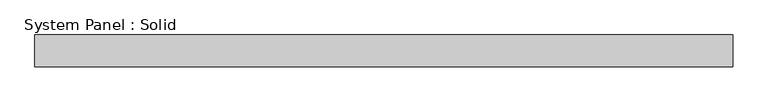
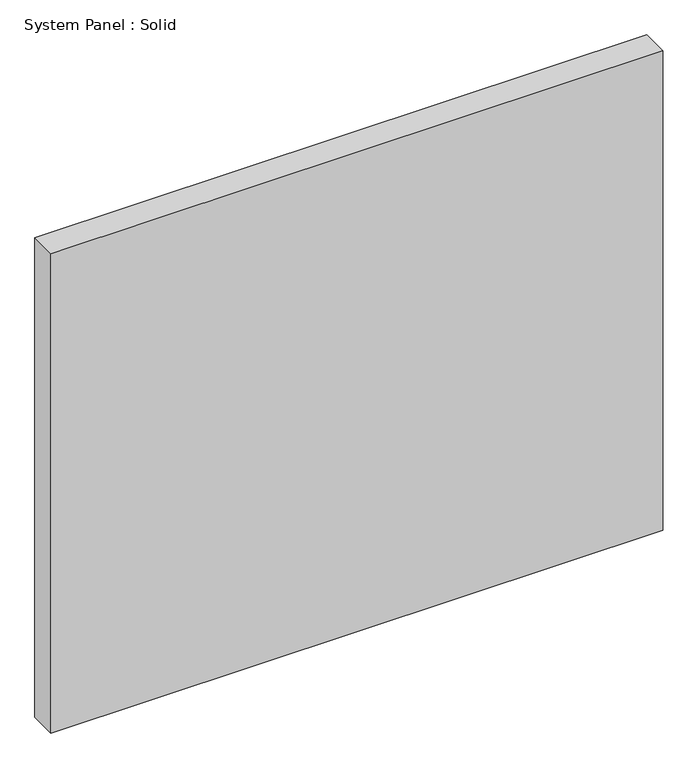
"""IFC4 building model written with IfcOpenShell, lengths in millimetres: plate geometry, System Panel : Solid."""

import ifcopenshell
import ifcopenshell.guid

model = None  # the IFC model being written
_history = None  # IfcOwnerHistory: only IFC2X3 demands one
_inside = {}  # id of a spatial element -> (the spatial element, [elements in it])
_under = {}  # id of a project, library or spatial element -> (it, [spatial elements below it])
_declared = {}  # id of a project -> (the project, [libraries it declares])
_typed = {}  # id of a type object -> (the type object, [elements of that type])
_made_of = {}  # id of a material, layer set ... -> (it, [elements and type objects made of it])


def new_model(schema):
    """Start an empty IFC model of exactly this schema.

    Asked for "IFC4X3", IfcOpenShell would pick the latest addendum, in which some entities
    have other attributes; the version numbers below select the first issue.
    IFC2X3 requires an IfcOwnerHistory on every rooted entity: one is made here for all.
    """
    global model, _history
    if schema == "IFC4X3":
        model = ifcopenshell.file(schema_version=(4, 3, 0, 0))
    else:
        model = ifcopenshell.file(schema=schema)
    _inside.clear()
    _under.clear()
    _declared.clear()
    _typed.clear()
    _made_of.clear()
    _history = None
    if model.schema == "IFC2X3":
        org = make("IfcOrganization", Name="unknown")
        user = make(
            "IfcPersonAndOrganization",
            ThePerson=make("IfcPerson", FamilyName="unknown"),
            TheOrganization=org,
        )
        app = make(
            "IfcApplication",
            ApplicationDeveloper=org,
            Version="unknown",
            ApplicationFullName="unknown",
            ApplicationIdentifier="unknown",
        )
        _history = make(
            "IfcOwnerHistory",
            OwningUser=user,
            OwningApplication=app,
            ChangeAction="ADDED",
            CreationDate=0,
        )
    return model


def make(cls, **values):
    """One entity of the class cls with the attributes given. An attribute that is None is left unset."""
    return model.create_entity(
        cls, **{name: value for name, value in values.items() if value is not None}
    )


def rooted(cls, **values):
    """An entity with a GlobalId (a new one), such as an element, a storey or a relation."""
    return make(cls, GlobalId=ifcopenshell.guid.new(), OwnerHistory=_history, **values)


def si_unit(unit_type, name, prefix=None):
    """IfcSIUnit, for example si_unit("LENGTHUNIT", "METRE", prefix="MILLI")."""
    return make("IfcSIUnit", UnitType=unit_type, Prefix=prefix, Name=name)


def assignment(units):
    """IfcUnitAssignment: the units of a project."""
    return None if units is None else make("IfcUnitAssignment", Units=units)


def point(xyz):
    """IfcCartesianPoint."""
    return None if xyz is None else make("IfcCartesianPoint", Coordinates=xyz)


def direction(xyz):
    """IfcDirection."""
    return None if xyz is None else make("IfcDirection", DirectionRatios=xyz)


def frame(location, z_axis=None, x_axis=None):
    """IfcAxis2Placement3D, a coordinate frame: its origin and axes. An axis left out is left unset."""
    return make(
        "IfcAxis2Placement3D",
        Location=point(location),
        Axis=direction(z_axis),
        RefDirection=direction(x_axis),
    )


def origin():
    """The frame at (0, 0, 0) with its axes left unset."""
    return frame((0.0, 0.0, 0.0))


def origin_with_axes():
    """The frame at (0, 0, 0) with the z axis (0, 0, 1) and the x axis (1, 0, 0) written out."""
    return frame((0.0, 0.0, 0.0), z_axis=(0.0, 0.0, 1.0), x_axis=(1.0, 0.0, 0.0))


def place(relative_to, where):
    """IfcLocalPlacement: puts the frame where relative to a parent placement (None: the world)."""
    return make(
        "IfcLocalPlacement", PlacementRelTo=relative_to, RelativePlacement=where
    )


def context(
    kind, dimensions, precision=None, world=None, true_north=None, identifier=None
):
    """IfcGeometricRepresentationContext, for example the 3D "Model" context."""
    return make(
        "IfcGeometricRepresentationContext",
        ContextIdentifier=identifier,
        ContextType=kind,
        CoordinateSpaceDimension=dimensions,
        Precision=precision,
        WorldCoordinateSystem=world,
        TrueNorth=true_north,
    )


def project(units=None, contexts=None):
    """IfcProject with its units and contexts."""
    return rooted(
        "IfcProject",
        Name="project",
        RepresentationContexts=contexts,
        UnitsInContext=assignment(units),
    )


def spatial(cls, under=None, at=None, **own):
    """A site, building, storey or space (cls), placed at a placement, below another one or the project."""
    s = rooted(cls, ObjectPlacement=at, **own)
    if under is not None:
        _under.setdefault(under.id(), (under, []))[1].append(s)
    return s


def polyline(points):
    """IfcPolyline through the points."""
    return make("IfcPolyline", Points=[point(p) for p in points])


def outline(outer, holes=None, kind="AREA"):
    """IfcArbitraryClosedProfileDef: a profile drawn as a closed curve; with holes, ...WithVoids."""
    if holes is None:
        return make("IfcArbitraryClosedProfileDef", ProfileType=kind, OuterCurve=outer)
    return make(
        "IfcArbitraryProfileDefWithVoids",
        ProfileType=kind,
        OuterCurve=outer,
        InnerCurves=holes,
    )


def extrude(swept, where, along, depth):
    """IfcExtrudedAreaSolid: the profile swept, set in the frame where, extruded along a direction by depth."""
    return make(
        "IfcExtrudedAreaSolid",
        SweptArea=swept,
        Position=where,
        ExtrudedDirection=direction(along),
        Depth=depth,
    )


def shape(context_of_items, identifier, shape_type, items):
    """IfcShapeRepresentation: the items that make up one representation, for example the "Body"."""
    return make(
        "IfcShapeRepresentation",
        ContextOfItems=context_of_items,
        RepresentationIdentifier=identifier,
        RepresentationType=shape_type,
        Items=items,
    )


def source(mapping_origin, context_of_items, identifier, shape_type, items):
    """IfcRepresentationMap: a shape defined once, which mapped items show again and again."""
    return make(
        "IfcRepresentationMap",
        MappingOrigin=mapping_origin,
        MappedRepresentation=shape(context_of_items, identifier, shape_type, items),
    )


def transform(
    local_origin,
    x_axis=None,
    y_axis=None,
    z_axis=None,
    scale=None,
    scale2=None,
    scale3=None,
    uniform=True,
):
    """IfcCartesianTransformationOperator3D, or its non-uniform kind. x_axis, y_axis, z_axis: its Axis1, 2, 3."""
    if uniform:
        return make(
            "IfcCartesianTransformationOperator3D",
            Axis1=direction(x_axis),
            Axis2=direction(y_axis),
            LocalOrigin=point(local_origin),
            Scale=scale,
            Axis3=direction(z_axis),
        )
    return make(
        "IfcCartesianTransformationOperator3DnonUniform",
        Axis1=direction(x_axis),
        Axis2=direction(y_axis),
        LocalOrigin=point(local_origin),
        Scale=scale,
        Axis3=direction(z_axis),
        Scale2=scale2,
        Scale3=scale3,
    )


def mapped(mapping_source, mapping_target):
    """IfcMappedItem: shows the shape of a source again, moved by a transform."""
    return make(
        "IfcMappedItem", MappingSource=mapping_source, MappingTarget=mapping_target
    )


def made_of(thing, what):
    """Note that an element or type object is made of a material, layer set ...; save() writes the relation."""
    if what is not None:
        _made_of.setdefault(what.id(), (what, []))[1].append(thing)
    return thing


def element(
    cls,
    number,
    at=None,
    inside=None,
    cuts=None,
    type_object=None,
    material=None,
    context=None,
    identifier="Body",
    shape_type=None,
    held_by="IfcProductDefinitionShape",
    body=None,
    shapes=None,
    **own,
):
    """One element of the class cls, such as IfcWall. Its Tag is "e" and its number.

    at: its placement. inside: the storey or other place that contains it. cuts: it is an
    opening in that element (IfcRelVoidsElement). A single representation is given by context,
    identifier, shape_type and body (its items); several are given by shapes. held_by: the class
    of the entity that holds the representations. save() writes the other relations.
    """
    e = rooted(cls, Tag="e%d" % number, ObjectPlacement=at, **own)
    if body is not None:
        shapes = [shape(context, identifier, shape_type, body)]
    if shapes is not None:
        e.Representation = make(held_by, Representations=shapes)
    if inside is not None:
        _inside.setdefault(inside.id(), (inside, []))[1].append(e)
    if cuts is not None:
        rooted(
            "IfcRelVoidsElement", RelatingBuildingElement=cuts, RelatedOpeningElement=e
        )
    if type_object is not None:
        _typed.setdefault(type_object.id(), (type_object, []))[1].append(e)
    return made_of(e, material)


def aggregate(whole, parts):
    """IfcRelAggregates: a whole, such as a stair, and the parts it consists of."""
    return rooted("IfcRelAggregates", RelatingObject=whole, RelatedObjects=parts)


def save(model, path):
    """Write the relations noted so far, then the file.

    IfcRelAggregates (storeys below a building ...), IfcRelContainedInSpatialStructure (elements
    in a storey), IfcRelDefinesByType, IfcRelAssociatesMaterial and IfcRelDeclares: one each for
    every whole, place, type object, material and project.
    """
    for whole, parts in _under.values():
        aggregate(whole, parts)
    for where, things in _inside.values():
        rooted(
            "IfcRelContainedInSpatialStructure",
            RelatedElements=things,
            RelatingStructure=where,
        )
    for kind, things in _typed.values():
        rooted("IfcRelDefinesByType", RelatedObjects=things, RelatingType=kind)
    for what, things in _made_of.values():
        rooted("IfcRelAssociatesMaterial", RelatedObjects=things, RelatingMaterial=what)
    for by, libraries in _declared.values():
        rooted("IfcRelDeclares", RelatingContext=by, RelatedDefinitions=libraries)
    model.write(path)


def system_panel_solid_99af49ff(model_context):
    return source(origin(), model_context, "Body", "SweptSolid", [
        extrude(outline(polyline([(697.4416668, -44.45), (-697.4416668, -44.45), (-697.4416668, 19.05), (697.4416668, 19.05), (697.4416668, -44.45)])), origin_with_axes(), (0.0, 0.0, 1.0), 1155.7),
    ])


if __name__ == "__main__":
    model = new_model("IFC4")
    model_context = context("Model", 3, world=origin())
    ifc_project = project(units=[si_unit("LENGTHUNIT", "METRE", prefix="MILLI")], contexts=[model_context])
    site = spatial("IfcSite", under=ifc_project)
    building = spatial("IfcBuilding", under=site)
    placement = place(None, origin())
    system_panel_solid_shape = system_panel_solid_99af49ff(model_context)
    element("IfcPlate", 1, ObjectType="System Panel : Solid", at=placement, inside=building, context=model_context, shape_type="MappedRepresentation", body=[
        mapped(system_panel_solid_shape, transform((0.0, 0.0, 0.0), x_axis=(1.0, 0.0, 0.0), y_axis=(0.0, 1.0, 0.0), z_axis=(0.0, 0.0, 1.0))),
    ])
    save(model, "model.ifc")

# Revit data of these elements
# Type "System Panel : Solid"
#   Construction Type Id = "MDOOR"
#   Analytic Construction = "Metal"
#   Visual Light Transmittance = 0
#   Solar Heat Gain Coefficient = 0
#   Heat Transfer Coefficient (U) = 0.651978 BTU/(h·ft²·°F)
#   Define Thermal Properties by = 1
# Element 1 (IfcPlate, "System Panel : Solid")
#   Materials on its faces: "Default"
# Materials
#   "Default": class "Miscellaneous", colour RGB 127 127 127, transparency 0, Cost = 0
